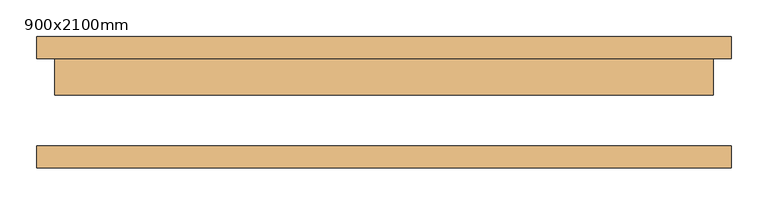
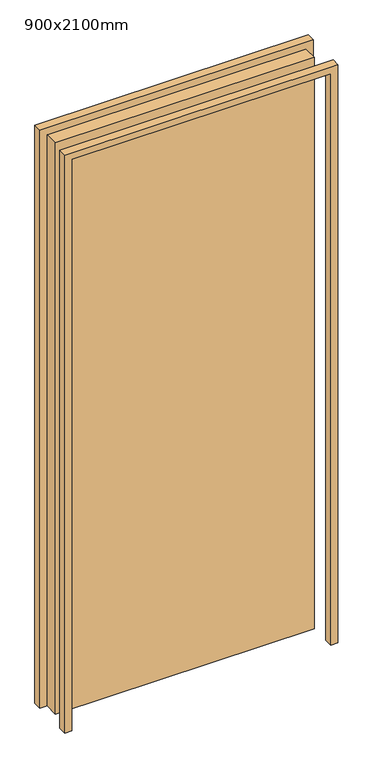
"""IFC4 building model written with IfcOpenShell, lengths in millimetres: door geometry, WWm-SingleSolid-Flush : 900x2100mm."""

from ifc_helpers import new_model, si_unit, frame, origin, origin_with_axes, place, context, project, spatial, polyline, outline, extrude, source, transform, mapped, element, save


def door_900x2100mm_c471ec78(model_context):
    return source(origin(), model_context, "Body", "SweptSolid", [
        extrude(outline(polyline([(2125.0, -475.0), (0.0, -475.0), (0.0, -450.0), (2100.0, -450.0), (2100.0, 450.0), (0.0, 450.0), (0.0, 475.0), (2125.0, 475.0), (2125.0, -475.0)])), frame((0.0, 60.0, 0.0), z_axis=(0.0, 1.0, 0.0), x_axis=(0.0, 0.0, 1.0)), (0.0, 0.0, 1.0), 30.0),
        extrude(outline(polyline([(2125.0, 475.0), (2125.0, -475.0), (0.0, -475.0), (0.0, -450.0), (2100.0, -450.0), (2100.0, 450.0), (0.0, 450.0), (0.0, 475.0), (2125.0, 475.0)])), frame((0.0, -90.0, 0.0), z_axis=(0.0, 1.0, 0.0), x_axis=(0.0, 0.0, 1.0)), (0.0, 0.0, 1.0), 30.0),
        extrude(outline(polyline([(450.0, 10.0), (-450.0, 10.0), (-450.0, 60.0), (450.0, 60.0), (450.0, 10.0)])), origin_with_axes(), (0.0, 0.0, 1.0), 2100.0),
    ])


if __name__ == "__main__":
    model = new_model("IFC4")
    model_context = context("Model", 3, world=origin())
    ifc_project = project(units=[si_unit("LENGTHUNIT", "METRE", prefix="MILLI")], contexts=[model_context])
    site = spatial("IfcSite", under=ifc_project)
    building = spatial("IfcBuilding", under=site)
    placement = place(None, origin())
    door_900x2100mm_shape = door_900x2100mm_c471ec78(model_context)
    element("IfcDoor", 1, ObjectType="WWm-SingleSolid-Flush : 900x2100mm", at=placement, inside=building, context=model_context, shape_type="MappedRepresentation", body=[
        mapped(door_900x2100mm_shape, transform((0.0, 0.0, 0.0), x_axis=(1.0, 0.0, 0.0), y_axis=(0.0, 1.0, 0.0), z_axis=(0.0, 0.0, 1.0))),
    ])
    save(model, "model.ifc")

# Revit data of these elements
# Type "WWm-SingleSolid-Flush : 900x2100mm"
#   Type Mark = "EX1-52"
#   Construction Type Id = "MDOOR"
#   Assembly Code = "C1020"
#   Analytic Construction = "Metal"
#   Thickness = 50 mm
#   Thermal Resistance (R) = 0.270117 (m²·K)/W
#   Heat Transfer Coefficient (U) = 3.7021 W/(m²·K)
#   Height = 2100 mm
#   Trim Projection Ext = 30 mm
#   Trim Projection Int = 30 mm
#   Trim Width = 25 mm
#   Width = 900 mm
#   Not 90 Degree [instance default] = no
#   90 Degree [instance default] = yes
#   Door Material = WW-EC-RGB-White
#   Frame Material = WW-EC-RGB-White
#   Visual Light Transmittance = 0
#   Solar Heat Gain Coefficient = 0
#   Function = (empty or 0)
#   Wall Closure = (empty or 0)
# Element 1 (IfcDoor, "WWm-SingleSolid-Flush : 900x2100mm")
#   Materials on its faces: "WW-EC-RGB-White"
# Materials
#   "WW-EC-RGB-White": class "Generic", colour RGB 255 255 255, transparency 0, Comments = "If region requests off-white, swith asset color to RGB 231-228-220", Description = "Generic Color", Cost = 0
